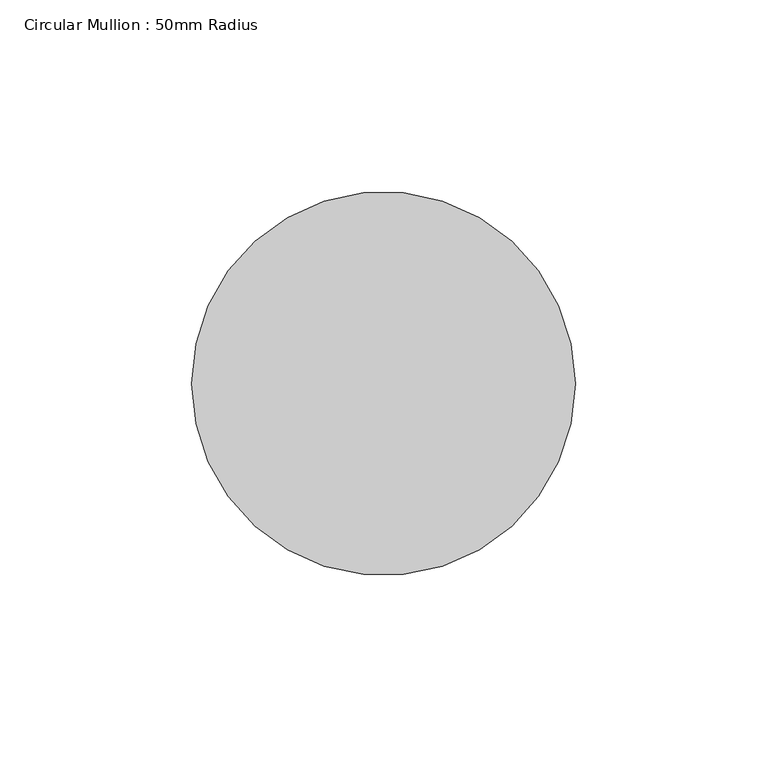
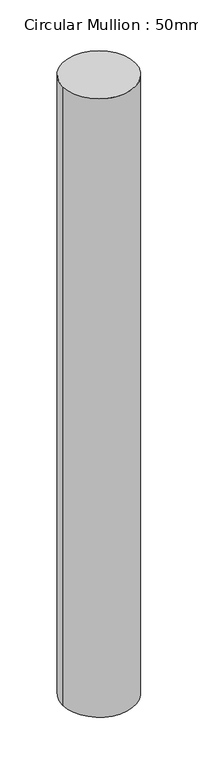
"""IFC4 building model written with IfcOpenShell, lengths in millimetres: member geometry, Circular Mullion : 50mm Radius."""

import ifcopenshell
import ifcopenshell.guid

model = None  # the IFC model being written
_history = None  # IfcOwnerHistory: only IFC2X3 demands one
_inside = {}  # id of a spatial element -> (the spatial element, [elements in it])
_under = {}  # id of a project, library or spatial element -> (it, [spatial elements below it])
_declared = {}  # id of a project -> (the project, [libraries it declares])
_typed = {}  # id of a type object -> (the type object, [elements of that type])
_made_of = {}  # id of a material, layer set ... -> (it, [elements and type objects made of it])


def new_model(schema):
    """Start an empty IFC model of exactly this schema.

    Asked for "IFC4X3", IfcOpenShell would pick the latest addendum, in which some entities
    have other attributes; the version numbers below select the first issue.
    IFC2X3 requires an IfcOwnerHistory on every rooted entity: one is made here for all.
    """
    global model, _history
    if schema == "IFC4X3":
        model = ifcopenshell.file(schema_version=(4, 3, 0, 0))
    else:
        model = ifcopenshell.file(schema=schema)
    _inside.clear()
    _under.clear()
    _declared.clear()
    _typed.clear()
    _made_of.clear()
    _history = None
    if model.schema == "IFC2X3":
        org = make("IfcOrganization", Name="unknown")
        user = make(
            "IfcPersonAndOrganization",
            ThePerson=make("IfcPerson", FamilyName="unknown"),
            TheOrganization=org,
        )
        app = make(
            "IfcApplication",
            ApplicationDeveloper=org,
            Version="unknown",
            ApplicationFullName="unknown",
            ApplicationIdentifier="unknown",
        )
        _history = make(
            "IfcOwnerHistory",
            OwningUser=user,
            OwningApplication=app,
            ChangeAction="ADDED",
            CreationDate=0,
        )
    return model


def make(cls, **values):
    """One entity of the class cls with the attributes given. An attribute that is None is left unset."""
    return model.create_entity(
        cls, **{name: value for name, value in values.items() if value is not None}
    )


def rooted(cls, **values):
    """An entity with a GlobalId (a new one), such as an element, a storey or a relation."""
    return make(cls, GlobalId=ifcopenshell.guid.new(), OwnerHistory=_history, **values)


def si_unit(unit_type, name, prefix=None):
    """IfcSIUnit, for example si_unit("LENGTHUNIT", "METRE", prefix="MILLI")."""
    return make("IfcSIUnit", UnitType=unit_type, Prefix=prefix, Name=name)


def assignment(units):
    """IfcUnitAssignment: the units of a project."""
    return None if units is None else make("IfcUnitAssignment", Units=units)


def point(xyz):
    """IfcCartesianPoint."""
    return None if xyz is None else make("IfcCartesianPoint", Coordinates=xyz)


def direction(xyz):
    """IfcDirection."""
    return None if xyz is None else make("IfcDirection", DirectionRatios=xyz)


def frame(location, z_axis=None, x_axis=None):
    """IfcAxis2Placement3D, a coordinate frame: its origin and axes. An axis left out is left unset."""
    return make(
        "IfcAxis2Placement3D",
        Location=point(location),
        Axis=direction(z_axis),
        RefDirection=direction(x_axis),
    )


def frame_2d(location, x_axis=None):
    """IfcAxis2Placement2D, a coordinate frame in the plane: its origin and x axis."""
    return make(
        "IfcAxis2Placement2D", Location=point(location), RefDirection=direction(x_axis)
    )


def origin():
    """The frame at (0, 0, 0) with its axes left unset."""
    return frame((0.0, 0.0, 0.0))


def origin_2d():
    """The frame at (0, 0) in the plane with its x axis left unset."""
    return frame_2d((0.0, 0.0))


def place(relative_to, where):
    """IfcLocalPlacement: puts the frame where relative to a parent placement (None: the world)."""
    return make(
        "IfcLocalPlacement", PlacementRelTo=relative_to, RelativePlacement=where
    )


def context(
    kind, dimensions, precision=None, world=None, true_north=None, identifier=None
):
    """IfcGeometricRepresentationContext, for example the 3D "Model" context."""
    return make(
        "IfcGeometricRepresentationContext",
        ContextIdentifier=identifier,
        ContextType=kind,
        CoordinateSpaceDimension=dimensions,
        Precision=precision,
        WorldCoordinateSystem=world,
        TrueNorth=true_north,
    )


def project(units=None, contexts=None):
    """IfcProject with its units and contexts."""
    return rooted(
        "IfcProject",
        Name="project",
        RepresentationContexts=contexts,
        UnitsInContext=assignment(units),
    )


def spatial(cls, under=None, at=None, **own):
    """A site, building, storey or space (cls), placed at a placement, below another one or the project."""
    s = rooted(cls, ObjectPlacement=at, **own)
    if under is not None:
        _under.setdefault(under.id(), (under, []))[1].append(s)
    return s


def circle_curve(where, radius):
    """IfcCircle in the frame where."""
    return make("IfcCircle", Position=where, Radius=radius)


def trimmed(basis, trim1, trim2, sense, master):
    """IfcTrimmedCurve: the piece of a basis curve between two trims."""
    return make(
        "IfcTrimmedCurve",
        BasisCurve=basis,
        Trim1=trim1,
        Trim2=trim2,
        SenseAgreement=sense,
        MasterRepresentation=master,
    )


def segment(curve, same_sense, transition):
    """IfcCompositeCurveSegment."""
    return make(
        "IfcCompositeCurveSegment",
        Transition=transition,
        SameSense=same_sense,
        ParentCurve=curve,
    )


def composite_curve(segments, self_intersect=None):
    """IfcCompositeCurve: segments joined end to end."""
    return make("IfcCompositeCurve", Segments=segments, SelfIntersect=self_intersect)


def outline(outer, holes=None, kind="AREA"):
    """IfcArbitraryClosedProfileDef: a profile drawn as a closed curve; with holes, ...WithVoids."""
    if holes is None:
        return make("IfcArbitraryClosedProfileDef", ProfileType=kind, OuterCurve=outer)
    return make(
        "IfcArbitraryProfileDefWithVoids",
        ProfileType=kind,
        OuterCurve=outer,
        InnerCurves=holes,
    )


def extrude(swept, where, along, depth):
    """IfcExtrudedAreaSolid: the profile swept, set in the frame where, extruded along a direction by depth."""
    return make(
        "IfcExtrudedAreaSolid",
        SweptArea=swept,
        Position=where,
        ExtrudedDirection=direction(along),
        Depth=depth,
    )


def shape(context_of_items, identifier, shape_type, items):
    """IfcShapeRepresentation: the items that make up one representation, for example the "Body"."""
    return make(
        "IfcShapeRepresentation",
        ContextOfItems=context_of_items,
        RepresentationIdentifier=identifier,
        RepresentationType=shape_type,
        Items=items,
    )


def source(mapping_origin, context_of_items, identifier, shape_type, items):
    """IfcRepresentationMap: a shape defined once, which mapped items show again and again."""
    return make(
        "IfcRepresentationMap",
        MappingOrigin=mapping_origin,
        MappedRepresentation=shape(context_of_items, identifier, shape_type, items),
    )


def transform(
    local_origin,
    x_axis=None,
    y_axis=None,
    z_axis=None,
    scale=None,
    scale2=None,
    scale3=None,
    uniform=True,
):
    """IfcCartesianTransformationOperator3D, or its non-uniform kind. x_axis, y_axis, z_axis: its Axis1, 2, 3."""
    if uniform:
        return make(
            "IfcCartesianTransformationOperator3D",
            Axis1=direction(x_axis),
            Axis2=direction(y_axis),
            LocalOrigin=point(local_origin),
            Scale=scale,
            Axis3=direction(z_axis),
        )
    return make(
        "IfcCartesianTransformationOperator3DnonUniform",
        Axis1=direction(x_axis),
        Axis2=direction(y_axis),
        LocalOrigin=point(local_origin),
        Scale=scale,
        Axis3=direction(z_axis),
        Scale2=scale2,
        Scale3=scale3,
    )


def mapped(mapping_source, mapping_target):
    """IfcMappedItem: shows the shape of a source again, moved by a transform."""
    return make(
        "IfcMappedItem", MappingSource=mapping_source, MappingTarget=mapping_target
    )


def made_of(thing, what):
    """Note that an element or type object is made of a material, layer set ...; save() writes the relation."""
    if what is not None:
        _made_of.setdefault(what.id(), (what, []))[1].append(thing)
    return thing


def element(
    cls,
    number,
    at=None,
    inside=None,
    cuts=None,
    type_object=None,
    material=None,
    context=None,
    identifier="Body",
    shape_type=None,
    held_by="IfcProductDefinitionShape",
    body=None,
    shapes=None,
    **own,
):
    """One element of the class cls, such as IfcWall. Its Tag is "e" and its number.

    at: its placement. inside: the storey or other place that contains it. cuts: it is an
    opening in that element (IfcRelVoidsElement). A single representation is given by context,
    identifier, shape_type and body (its items); several are given by shapes. held_by: the class
    of the entity that holds the representations. save() writes the other relations.
    """
    e = rooted(cls, Tag="e%d" % number, ObjectPlacement=at, **own)
    if body is not None:
        shapes = [shape(context, identifier, shape_type, body)]
    if shapes is not None:
        e.Representation = make(held_by, Representations=shapes)
    if inside is not None:
        _inside.setdefault(inside.id(), (inside, []))[1].append(e)
    if cuts is not None:
        rooted(
            "IfcRelVoidsElement", RelatingBuildingElement=cuts, RelatedOpeningElement=e
        )
    if type_object is not None:
        _typed.setdefault(type_object.id(), (type_object, []))[1].append(e)
    return made_of(e, material)


def aggregate(whole, parts):
    """IfcRelAggregates: a whole, such as a stair, and the parts it consists of."""
    return rooted("IfcRelAggregates", RelatingObject=whole, RelatedObjects=parts)


def save(model, path):
    """Write the relations noted so far, then the file.

    IfcRelAggregates (storeys below a building ...), IfcRelContainedInSpatialStructure (elements
    in a storey), IfcRelDefinesByType, IfcRelAssociatesMaterial and IfcRelDeclares: one each for
    every whole, place, type object, material and project.
    """
    for whole, parts in _under.values():
        aggregate(whole, parts)
    for where, things in _inside.values():
        rooted(
            "IfcRelContainedInSpatialStructure",
            RelatedElements=things,
            RelatingStructure=where,
        )
    for kind, things in _typed.values():
        rooted("IfcRelDefinesByType", RelatedObjects=things, RelatingType=kind)
    for what, things in _made_of.values():
        rooted("IfcRelAssociatesMaterial", RelatedObjects=things, RelatingMaterial=what)
    for by, libraries in _declared.values():
        rooted("IfcRelDeclares", RelatingContext=by, RelatedDefinitions=libraries)
    model.write(path)


def circular_mullion_50mm_radius_e2316d1f(model_context):
    return source(origin(), model_context, "Body", "SweptSolid", [
        extrude(outline(composite_curve([segment(trimmed(circle_curve(origin_2d(), 50.0), [point((50.0, 0.0))], [point((-50.0, 0.0))], False, "CARTESIAN"), True, "CONTINUOUS"), segment(trimmed(circle_curve(origin_2d(), 50.0), [point((-50.0, 0.0))], [point((50.0, 0.0))], False, "CARTESIAN"), True, "CONTINUOUS")], self_intersect=False)), frame((0.0, 0.0, -900.7355632), z_axis=(0.0, 0.0, 1.0), x_axis=(1.0, 0.0, 0.0)), (0.0, 0.0, 1.0), 900.7355632),
    ])


if __name__ == "__main__":
    model = new_model("IFC4")
    model_context = context("Model", 3, world=origin())
    ifc_project = project(units=[si_unit("LENGTHUNIT", "METRE", prefix="MILLI")], contexts=[model_context])
    site = spatial("IfcSite", under=ifc_project)
    building = spatial("IfcBuilding", under=site)
    placement = place(None, origin())
    circular_mullion_50mm_radius_shape = circular_mullion_50mm_radius_e2316d1f(model_context)
    element("IfcMember", 1, ObjectType="Circular Mullion : 50mm Radius", at=placement, inside=building, context=model_context, shape_type="MappedRepresentation", body=[
        mapped(circular_mullion_50mm_radius_shape, transform((0.0, 0.0, 0.0), x_axis=(1.0, 0.0, 0.0), y_axis=(0.0, 1.0, 0.0), z_axis=(0.0, 0.0, 1.0))),
    ])
    save(model, "model.ifc")

# Revit data of these elements
# Type "Circular Mullion : 50mm Radius"
#   built-in parameter 1007350 = 0.164042 (stored number, unit not read)
# Element 1 (IfcMember, "Circular Mullion : 50mm Radius")
#   Materials on its faces: "Aluminium"
# Materials
#   "Aluminium": class "Metal", colour RGB 247 247 247, transparency 0, Description = "Aluminium 6061", Cost = 0
